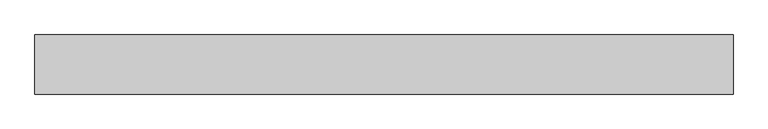
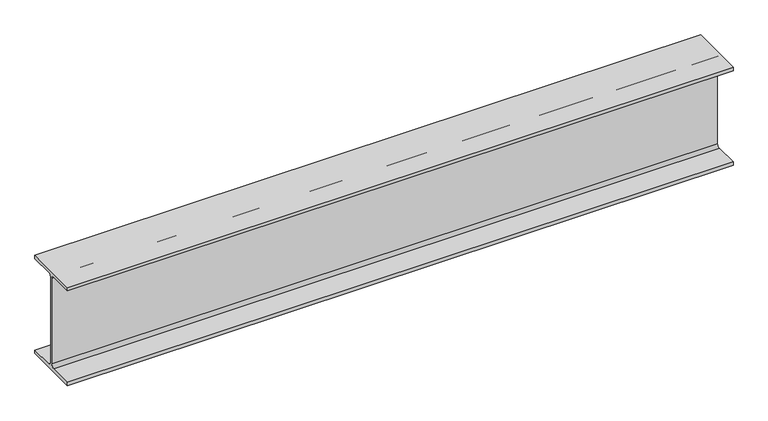
"""IFC4 building model written with IfcOpenShell, lengths in millimetres: beam geometry, Steel Beam_H-KSD3502 : H_SB_ASB_H-200x200x8x12."""

from ifc_helpers import new_model, si_unit, point, frame, frame_2d, origin, place, context, project, spatial, polyline, circle_curve, trimmed, segment, composite_curve, outline, extrude, source, transform, mapped, element, save


def beam_cc15ee5d(model_context):
    return source(origin(), model_context, "Body", "SweptSolid", [
        extrude(outline(composite_curve([segment(polyline([(82.5, -141.5), (82.5, -151.7), (-82.5, -151.7), (-82.5, -141.5), (-11.9, -141.5)]), True, "CONTINUOUS"), segment(trimmed(circle_curve(frame_2d((-11.9, -132.6)), 8.9), [point((-11.9, -141.5))], [point((-3.0, -132.6))], True, "CARTESIAN"), True, "CONTINUOUS"), segment(polyline([(-3.0, -132.6), (-3.0, 132.6)]), True, "CONTINUOUS"), segment(trimmed(circle_curve(frame_2d((-11.9, 132.6)), 8.9), [point((-3.0, 132.6))], [point((-11.9, 141.5))], True, "CARTESIAN"), True, "CONTINUOUS"), segment(polyline([(-11.9, 141.5), (-82.5, 141.5), (-82.5, 151.7), (82.5, 151.7), (82.5, 141.5), (11.9, 141.5)]), True, "CONTINUOUS"), segment(trimmed(circle_curve(frame_2d((11.9, 132.6)), 8.9), [point((11.9, 141.5))], [point((3.0, 132.6))], True, "CARTESIAN"), True, "CONTINUOUS"), segment(polyline([(3.0, 132.6), (3.0, -132.6)]), True, "CONTINUOUS"), segment(trimmed(circle_curve(frame_2d((11.9, -132.6)), 8.9), [point((3.0, -132.6))], [point((11.9, -141.5))], True, "CARTESIAN"), True, "CONTINUOUS"), segment(polyline([(11.9, -141.5), (82.5, -141.5)]), True, "CONTINUOUS")], self_intersect=False)), frame((-921.1968525, 0.0, 0.0), z_axis=(1.0, 0.0, 0.0), x_axis=(0.0, 1.0, 0.0)), (0.0, 0.0, 1.0), 1948.528739),
    ])


if __name__ == "__main__":
    model = new_model("IFC4")
    model_context = context("Model", 3, world=origin())
    ifc_project = project(units=[si_unit("LENGTHUNIT", "METRE", prefix="MILLI")], contexts=[model_context])
    site = spatial("IfcSite", under=ifc_project)
    building = spatial("IfcBuilding", under=site)
    placement = place(None, origin())
    beam_shape = beam_cc15ee5d(model_context)
    element("IfcBeam", 1, ObjectType="Steel Beam_H-KSD3502 : H_SB_ASB_H-200x200x8x12", at=placement, inside=building, context=model_context, shape_type="MappedRepresentation", body=[
        mapped(beam_shape, transform((0.0, 0.0, 0.0), x_axis=(1.0, 0.0, 0.0), y_axis=(0.0, 1.0, 0.0), z_axis=(0.0, 0.0, 1.0))),
    ])
    save(model, "model.ifc")

# Revit data of these elements
# Type "Steel Beam_H-KSD3502 : H_SB_ASB_H-200x200x8x12"
#   Width = 20.0 cm
#   Web Thickness = 0.8 cm
#   Web Fillet = 1.3 cm
#   Warping Constant = 141376.0 cm⁶
#   Torsional Moment of Inertia = 26.2485 cm⁴
#   Torsional Modulus = 1.0 cm³
#   Section Area = 63.53 cm²
#   Plastic Modulus weak axis = 244.0 cm³
#   Plastic Modulus strong axis = 525.0 cm³
#   Perimeter = 1.16 m²/m
#   Nominal Weight = 49.90 kgf/m
#   Moment of Inertia weak axis = 1600.00 cm⁴
#   Moment of Inertia strong axis = 4720.00 cm⁴
#   Height = 20.0 cm
#   Flange Thickness = 1.2 cm
#   Elastic Modulus weak axis = 160.0 cm³
#   Elastic Modulus strong axis = 472.0 cm³
#   Centroid Vertical = 10.0 cm
#   Centroid Horizontal = 10.0 cm
#   Length [instance default] = 1.5240 m
#   Structural Material [instance default] = Steel, 45-345
#   Assembly Code = ""
# Element 1 (IfcBeam, "Steel Beam_H-KSD3502 : H_SB_ASB_H-200x200x8x12")
#   Structural Material = none
# Materials
#   "Steel, 45-345": class "Metal", colour RGB 189 187 185, transparency 0, Description = "Steel 345 MPa", Cost = 0
